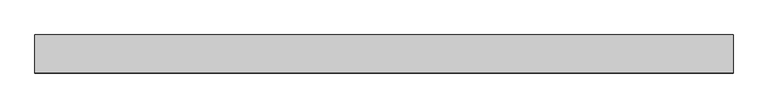
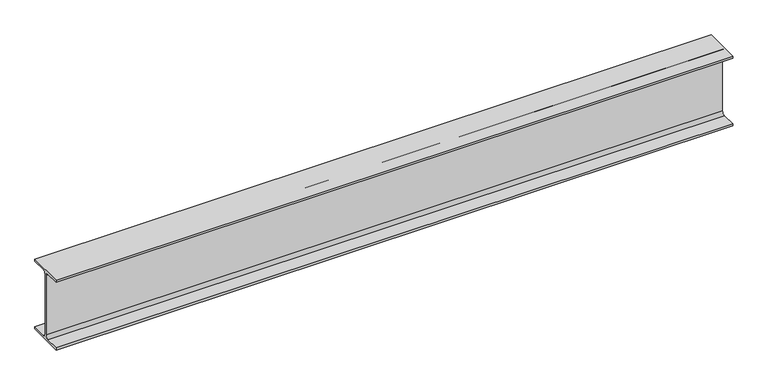
"""IFC4 building model written with IfcOpenShell, lengths in millimetres: beam geometry, Steel Framing_H_KS : H_SB_AR_S02_H-300x150x6.5x9_WG1."""

from ifc_helpers import new_model, si_unit, point, frame, frame_2d, origin, place, context, project, spatial, polyline, circle_curve, trimmed, segment, composite_curve, outline, extrude, source, transform, mapped, element, save


def beam_78b55b0a(model_context):
    return source(origin(), model_context, "Body", "SweptSolid", [
        extrude(outline(composite_curve([segment(polyline([(75.0, -141.0), (75.0, -150.0), (-75.0, -150.0), (-75.0, -141.0), (-16.25, -141.0)]), True, "CONTINUOUS"), segment(trimmed(circle_curve(frame_2d((-16.25, -128.0)), 13.0), [point((-16.25, -141.0))], [point((-3.25, -128.0))], True, "CARTESIAN"), True, "CONTINUOUS"), segment(polyline([(-3.25, -128.0), (-3.25, 128.0)]), True, "CONTINUOUS"), segment(trimmed(circle_curve(frame_2d((-16.25, 128.0)), 13.0), [point((-3.25, 128.0))], [point((-16.25, 141.0))], True, "CARTESIAN"), True, "CONTINUOUS"), segment(polyline([(-16.25, 141.0), (-75.0, 141.0), (-75.0, 150.0), (75.0, 150.0), (75.0, 141.0), (16.25, 141.0)]), True, "CONTINUOUS"), segment(trimmed(circle_curve(frame_2d((16.25, 128.0)), 13.0), [point((16.25, 141.0))], [point((3.25, 128.0))], True, "CARTESIAN"), True, "CONTINUOUS"), segment(polyline([(3.25, 128.0), (3.25, -128.0)]), True, "CONTINUOUS"), segment(trimmed(circle_curve(frame_2d((16.25, -128.0)), 13.0), [point((3.25, -128.0))], [point((16.25, -141.0))], True, "CARTESIAN"), True, "CONTINUOUS"), segment(polyline([(16.25, -141.0), (75.0, -141.0)]), True, "CONTINUOUS")], self_intersect=False)), frame((-1337.3, 0.0, 0.0), z_axis=(1.0, 0.0, 0.0), x_axis=(0.0, 1.0, 0.0)), (0.0, 0.0, 1.0), 2749.6),
    ])


if __name__ == "__main__":
    model = new_model("IFC4")
    model_context = context("Model", 3, world=origin())
    ifc_project = project(units=[si_unit("LENGTHUNIT", "METRE", prefix="MILLI")], contexts=[model_context])
    site = spatial("IfcSite", under=ifc_project)
    building = spatial("IfcBuilding", under=site)
    placement = place(None, origin())
    beam_shape = beam_78b55b0a(model_context)
    element("IfcBeam", 1, ObjectType="Steel Framing_H_KS : H_SB_AR_S02_H-300x150x6.5x9_WG1", at=placement, inside=building, context=model_context, shape_type="MappedRepresentation", body=[
        mapped(beam_shape, transform((0.0, 0.0, 0.0), x_axis=(1.0, 0.0, 0.0), y_axis=(0.0, 1.0, 0.0), z_axis=(0.0, 0.0, 1.0))),
    ])
    save(model, "model.ifc")

# Revit data of these elements
# Type "Steel Framing_H_KS : H_SB_AR_S02_H-300x150x6.5x9_WG1"
#   Type Comments = "MAIN"
#   Type Mark = "WG1"
#   H_SectionID = "H-300x150x6.5x9"
#   H_Ratio for Additional Steel Plate = 0.2
#   Width = 15.0 cm
#   Web Thickness = 0.65 cm
#   Web Fillet = 1.3 cm
#   Warping Constant = 107000.0 cm⁶
#   Torsional Moment of Inertia = 9.9539 cm⁴
#   Section Area = 46.78 cm²
#   Plastic Modulus weak axis = 105.0 cm³
#   Plastic Modulus strong axis = 542.0 cm³
#   Perimeter = 1.17 m²/m
#   Nominal Weight = 36.70 kgf/m
#   Moment of Inertia weak axis = 508.00 cm⁴
#   Moment of Inertia strong axis = 7210.00 cm⁴
#   Height = 30.0 cm
#   Flange Thickness = 0.9 cm
#   Elastic Modulus weak axis = 67.7 cm³
#   Elastic Modulus strong axis = 481.0 cm³
#   Centroid Vertical = 15.0 cm
#   Centroid Horizontal = 7.5 cm
#   Bolt Spacing = 8.89 cm
#   Length [instance default] = 1500 mm
#   Structural Material [instance default] = Steel, 45-345
#   Section Name Key = ""
#   Assembly Code = ""
# Element 1 (IfcBeam, "Steel Framing_H_KS : H_SB_AR_S02_H-300x150x6.5x9_WG1")
#   Materials on its faces: "Steel, 45-345"
# Materials
#   "Steel, 45-345": class "Metal", colour RGB 189 187 185, transparency 0, Description = "Steel 345 MPa", Cost = 0
